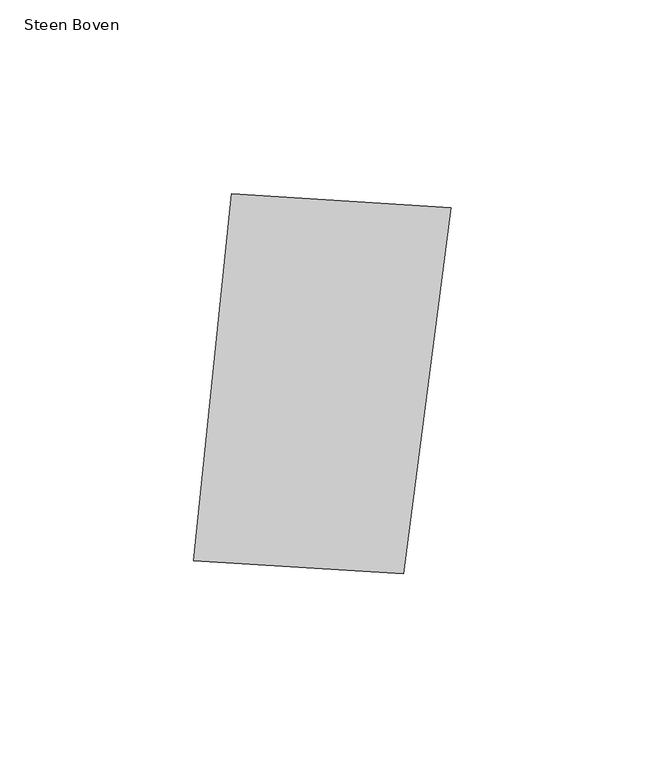
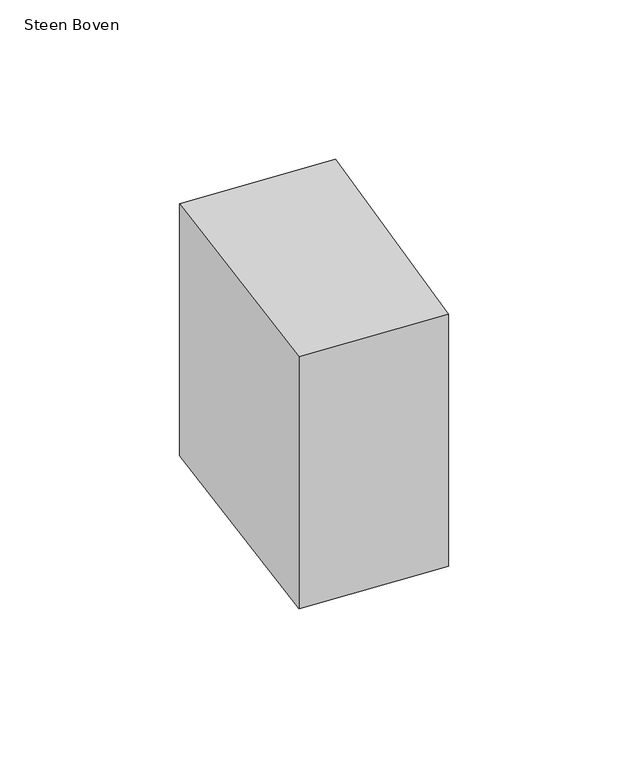
"""IFC4 building model written with IfcOpenShell, lengths in millimetres: proxy geometry, 00_GMA_steen_versie_4 : Steen Boven."""

from ifc_helpers import new_model, si_unit, origin, origin_with_axes, place, context, project, spatial, polyline, outline, extrude, source, transform, mapped, element, save


def steen_boven_456b610d(model_context):
    return source(origin(), model_context, "Body", "SweptSolid", [
        extrude(outline(polyline([(107.0099138, 118.6028536), (94.7591476, 24.1727813), (40.732272, 27.5568472), (50.4536922, 122.1390822), (107.0099138, 118.6028536)])), origin_with_axes(), (0.0, 0.0, 1.0), 100.0),
    ])


if __name__ == "__main__":
    model = new_model("IFC4")
    model_context = context("Model", 3, world=origin())
    ifc_project = project(units=[si_unit("LENGTHUNIT", "METRE", prefix="MILLI")], contexts=[model_context])
    site = spatial("IfcSite", under=ifc_project)
    building = spatial("IfcBuilding", under=site)
    placement = place(None, origin())
    steen_boven_shape = steen_boven_456b610d(model_context)
    element("IfcBuildingElementProxy", 1, Name="00_GMA_steen_versie_4 : Steen Boven", ObjectType="00_GMA_steen_versie_4 : Steen Boven", at=placement, inside=building, context=model_context, shape_type="MappedRepresentation", body=[
        mapped(steen_boven_shape, transform((0.0, 0.0, 0.0), x_axis=(1.0, 0.0, 0.0), y_axis=(0.0, 1.0, 0.0), z_axis=(0.0, 0.0, 1.0))),
    ])
    save(model, "model.ifc")

# Revit data of these elements
# Type "00_GMA_steen_versie_4 : Steen Boven"
#   StootVoegHalfBoven [instance default] = 5 mm
#   StootVoegHalf [instance default] = 5 mm
#   StootVoegBreedteOnder = 10 mm
#   StootVoegBreedteBoven = 10 mm
#   Steendikte = 100 mm
#   LintVoegOnderHalf = 5 mm
#   LintVoegOnder = 10 mm
#   LintVoegBovenHalf = 0 mm
#   LintVoegBoven = 0 mm
#   materiaal = none
#   MateriaalVoeg = none
#   Default Elevation = 0
